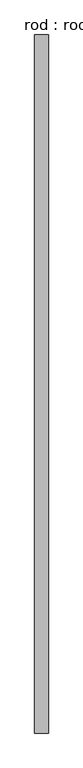
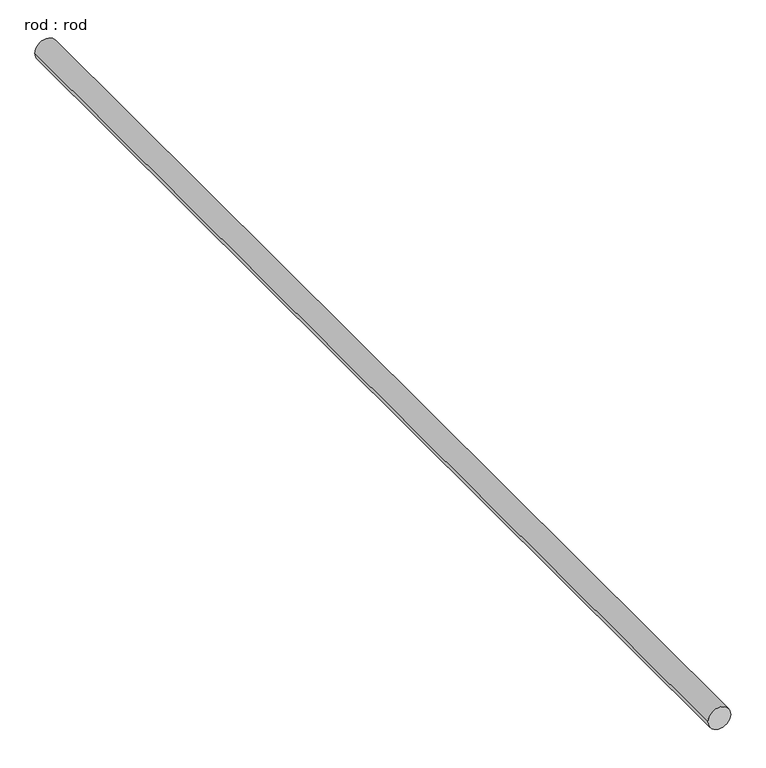
"""IFC4 building model written with IfcOpenShell, lengths in millimetres: proxy geometry, rod : rod."""

import ifcopenshell
import ifcopenshell.guid

model = None  # the IFC model being written
_history = None  # IfcOwnerHistory: only IFC2X3 demands one
_inside = {}  # id of a spatial element -> (the spatial element, [elements in it])
_under = {}  # id of a project, library or spatial element -> (it, [spatial elements below it])
_declared = {}  # id of a project -> (the project, [libraries it declares])
_typed = {}  # id of a type object -> (the type object, [elements of that type])
_made_of = {}  # id of a material, layer set ... -> (it, [elements and type objects made of it])


def new_model(schema):
    """Start an empty IFC model of exactly this schema.

    Asked for "IFC4X3", IfcOpenShell would pick the latest addendum, in which some entities
    have other attributes; the version numbers below select the first issue.
    IFC2X3 requires an IfcOwnerHistory on every rooted entity: one is made here for all.
    """
    global model, _history
    if schema == "IFC4X3":
        model = ifcopenshell.file(schema_version=(4, 3, 0, 0))
    else:
        model = ifcopenshell.file(schema=schema)
    _inside.clear()
    _under.clear()
    _declared.clear()
    _typed.clear()
    _made_of.clear()
    _history = None
    if model.schema == "IFC2X3":
        org = make("IfcOrganization", Name="unknown")
        user = make(
            "IfcPersonAndOrganization",
            ThePerson=make("IfcPerson", FamilyName="unknown"),
            TheOrganization=org,
        )
        app = make(
            "IfcApplication",
            ApplicationDeveloper=org,
            Version="unknown",
            ApplicationFullName="unknown",
            ApplicationIdentifier="unknown",
        )
        _history = make(
            "IfcOwnerHistory",
            OwningUser=user,
            OwningApplication=app,
            ChangeAction="ADDED",
            CreationDate=0,
        )
    return model


def make(cls, **values):
    """One entity of the class cls with the attributes given. An attribute that is None is left unset."""
    return model.create_entity(
        cls, **{name: value for name, value in values.items() if value is not None}
    )


def rooted(cls, **values):
    """An entity with a GlobalId (a new one), such as an element, a storey or a relation."""
    return make(cls, GlobalId=ifcopenshell.guid.new(), OwnerHistory=_history, **values)


def si_unit(unit_type, name, prefix=None):
    """IfcSIUnit, for example si_unit("LENGTHUNIT", "METRE", prefix="MILLI")."""
    return make("IfcSIUnit", UnitType=unit_type, Prefix=prefix, Name=name)


def assignment(units):
    """IfcUnitAssignment: the units of a project."""
    return None if units is None else make("IfcUnitAssignment", Units=units)


def point(xyz):
    """IfcCartesianPoint."""
    return None if xyz is None else make("IfcCartesianPoint", Coordinates=xyz)


def direction(xyz):
    """IfcDirection."""
    return None if xyz is None else make("IfcDirection", DirectionRatios=xyz)


def frame(location, z_axis=None, x_axis=None):
    """IfcAxis2Placement3D, a coordinate frame: its origin and axes. An axis left out is left unset."""
    return make(
        "IfcAxis2Placement3D",
        Location=point(location),
        Axis=direction(z_axis),
        RefDirection=direction(x_axis),
    )


def frame_2d(location, x_axis=None):
    """IfcAxis2Placement2D, a coordinate frame in the plane: its origin and x axis."""
    return make(
        "IfcAxis2Placement2D", Location=point(location), RefDirection=direction(x_axis)
    )


def origin():
    """The frame at (0, 0, 0) with its axes left unset."""
    return frame((0.0, 0.0, 0.0))


def place(relative_to, where):
    """IfcLocalPlacement: puts the frame where relative to a parent placement (None: the world)."""
    return make(
        "IfcLocalPlacement", PlacementRelTo=relative_to, RelativePlacement=where
    )


def context(
    kind, dimensions, precision=None, world=None, true_north=None, identifier=None
):
    """IfcGeometricRepresentationContext, for example the 3D "Model" context."""
    return make(
        "IfcGeometricRepresentationContext",
        ContextIdentifier=identifier,
        ContextType=kind,
        CoordinateSpaceDimension=dimensions,
        Precision=precision,
        WorldCoordinateSystem=world,
        TrueNorth=true_north,
    )


def project(units=None, contexts=None):
    """IfcProject with its units and contexts."""
    return rooted(
        "IfcProject",
        Name="project",
        RepresentationContexts=contexts,
        UnitsInContext=assignment(units),
    )


def spatial(cls, under=None, at=None, **own):
    """A site, building, storey or space (cls), placed at a placement, below another one or the project."""
    s = rooted(cls, ObjectPlacement=at, **own)
    if under is not None:
        _under.setdefault(under.id(), (under, []))[1].append(s)
    return s


def circle_curve(where, radius):
    """IfcCircle in the frame where."""
    return make("IfcCircle", Position=where, Radius=radius)


def trimmed(basis, trim1, trim2, sense, master):
    """IfcTrimmedCurve: the piece of a basis curve between two trims."""
    return make(
        "IfcTrimmedCurve",
        BasisCurve=basis,
        Trim1=trim1,
        Trim2=trim2,
        SenseAgreement=sense,
        MasterRepresentation=master,
    )


def segment(curve, same_sense, transition):
    """IfcCompositeCurveSegment."""
    return make(
        "IfcCompositeCurveSegment",
        Transition=transition,
        SameSense=same_sense,
        ParentCurve=curve,
    )


def composite_curve(segments, self_intersect=None):
    """IfcCompositeCurve: segments joined end to end."""
    return make("IfcCompositeCurve", Segments=segments, SelfIntersect=self_intersect)


def outline(outer, holes=None, kind="AREA"):
    """IfcArbitraryClosedProfileDef: a profile drawn as a closed curve; with holes, ...WithVoids."""
    if holes is None:
        return make("IfcArbitraryClosedProfileDef", ProfileType=kind, OuterCurve=outer)
    return make(
        "IfcArbitraryProfileDefWithVoids",
        ProfileType=kind,
        OuterCurve=outer,
        InnerCurves=holes,
    )


def extrude(swept, where, along, depth):
    """IfcExtrudedAreaSolid: the profile swept, set in the frame where, extruded along a direction by depth."""
    return make(
        "IfcExtrudedAreaSolid",
        SweptArea=swept,
        Position=where,
        ExtrudedDirection=direction(along),
        Depth=depth,
    )


def shape(context_of_items, identifier, shape_type, items):
    """IfcShapeRepresentation: the items that make up one representation, for example the "Body"."""
    return make(
        "IfcShapeRepresentation",
        ContextOfItems=context_of_items,
        RepresentationIdentifier=identifier,
        RepresentationType=shape_type,
        Items=items,
    )


def source(mapping_origin, context_of_items, identifier, shape_type, items):
    """IfcRepresentationMap: a shape defined once, which mapped items show again and again."""
    return make(
        "IfcRepresentationMap",
        MappingOrigin=mapping_origin,
        MappedRepresentation=shape(context_of_items, identifier, shape_type, items),
    )


def transform(
    local_origin,
    x_axis=None,
    y_axis=None,
    z_axis=None,
    scale=None,
    scale2=None,
    scale3=None,
    uniform=True,
):
    """IfcCartesianTransformationOperator3D, or its non-uniform kind. x_axis, y_axis, z_axis: its Axis1, 2, 3."""
    if uniform:
        return make(
            "IfcCartesianTransformationOperator3D",
            Axis1=direction(x_axis),
            Axis2=direction(y_axis),
            LocalOrigin=point(local_origin),
            Scale=scale,
            Axis3=direction(z_axis),
        )
    return make(
        "IfcCartesianTransformationOperator3DnonUniform",
        Axis1=direction(x_axis),
        Axis2=direction(y_axis),
        LocalOrigin=point(local_origin),
        Scale=scale,
        Axis3=direction(z_axis),
        Scale2=scale2,
        Scale3=scale3,
    )


def mapped(mapping_source, mapping_target):
    """IfcMappedItem: shows the shape of a source again, moved by a transform."""
    return make(
        "IfcMappedItem", MappingSource=mapping_source, MappingTarget=mapping_target
    )


def made_of(thing, what):
    """Note that an element or type object is made of a material, layer set ...; save() writes the relation."""
    if what is not None:
        _made_of.setdefault(what.id(), (what, []))[1].append(thing)
    return thing


def element(
    cls,
    number,
    at=None,
    inside=None,
    cuts=None,
    type_object=None,
    material=None,
    context=None,
    identifier="Body",
    shape_type=None,
    held_by="IfcProductDefinitionShape",
    body=None,
    shapes=None,
    **own,
):
    """One element of the class cls, such as IfcWall. Its Tag is "e" and its number.

    at: its placement. inside: the storey or other place that contains it. cuts: it is an
    opening in that element (IfcRelVoidsElement). A single representation is given by context,
    identifier, shape_type and body (its items); several are given by shapes. held_by: the class
    of the entity that holds the representations. save() writes the other relations.
    """
    e = rooted(cls, Tag="e%d" % number, ObjectPlacement=at, **own)
    if body is not None:
        shapes = [shape(context, identifier, shape_type, body)]
    if shapes is not None:
        e.Representation = make(held_by, Representations=shapes)
    if inside is not None:
        _inside.setdefault(inside.id(), (inside, []))[1].append(e)
    if cuts is not None:
        rooted(
            "IfcRelVoidsElement", RelatingBuildingElement=cuts, RelatedOpeningElement=e
        )
    if type_object is not None:
        _typed.setdefault(type_object.id(), (type_object, []))[1].append(e)
    return made_of(e, material)


def aggregate(whole, parts):
    """IfcRelAggregates: a whole, such as a stair, and the parts it consists of."""
    return rooted("IfcRelAggregates", RelatingObject=whole, RelatedObjects=parts)


def save(model, path):
    """Write the relations noted so far, then the file.

    IfcRelAggregates (storeys below a building ...), IfcRelContainedInSpatialStructure (elements
    in a storey), IfcRelDefinesByType, IfcRelAssociatesMaterial and IfcRelDeclares: one each for
    every whole, place, type object, material and project.
    """
    for whole, parts in _under.values():
        aggregate(whole, parts)
    for where, things in _inside.values():
        rooted(
            "IfcRelContainedInSpatialStructure",
            RelatedElements=things,
            RelatingStructure=where,
        )
    for kind, things in _typed.values():
        rooted("IfcRelDefinesByType", RelatedObjects=things, RelatingType=kind)
    for what, things in _made_of.values():
        rooted("IfcRelAssociatesMaterial", RelatedObjects=things, RelatingMaterial=what)
    for by, libraries in _declared.values():
        rooted("IfcRelDeclares", RelatingContext=by, RelatedDefinitions=libraries)
    model.write(path)


def rod_rod_5db25ccb(model_context):
    return source(origin(), model_context, "Body", "SweptSolid", [
        extrude(outline(composite_curve([segment(trimmed(circle_curve(frame_2d((0.0108462, 0.0)), 200.0), [point((0.0108462, 200.0))], [point((0.0108462, -200.0))], False, "CARTESIAN"), True, "CONTINUOUS"), segment(trimmed(circle_curve(frame_2d((0.0108462, 0.0)), 200.0), [point((0.0108462, -200.0))], [point((0.0108462, 200.0))], False, "CARTESIAN"), True, "CONTINUOUS")], self_intersect=False)), frame((0.0, -6124.9292774, 0.0), z_axis=(0.0, 1.0, 0.0), x_axis=(0.0, 0.0, 1.0)), (0.0, 0.0, 1.0), 20435.3157854),
    ])


if __name__ == "__main__":
    model = new_model("IFC4")
    model_context = context("Model", 3, world=origin())
    ifc_project = project(units=[si_unit("LENGTHUNIT", "METRE", prefix="MILLI")], contexts=[model_context])
    site = spatial("IfcSite", under=ifc_project)
    building = spatial("IfcBuilding", under=site)
    placement = place(None, origin())
    rod_rod_shape = rod_rod_5db25ccb(model_context)
    element("IfcBuildingElementProxy", 1, Name="rod : rod", ObjectType="rod : rod", at=placement, inside=building, context=model_context, shape_type="MappedRepresentation", body=[
        mapped(rod_rod_shape, transform((0.0, 0.0, 0.0), x_axis=(1.0, 0.0, 0.0), y_axis=(0.0, 1.0, 0.0), z_axis=(0.0, 0.0, 1.0))),
    ])
    save(model, "model.ifc")

# Revit data of these elements
# Type "rod : rod"
#   Default Elevation = 0
